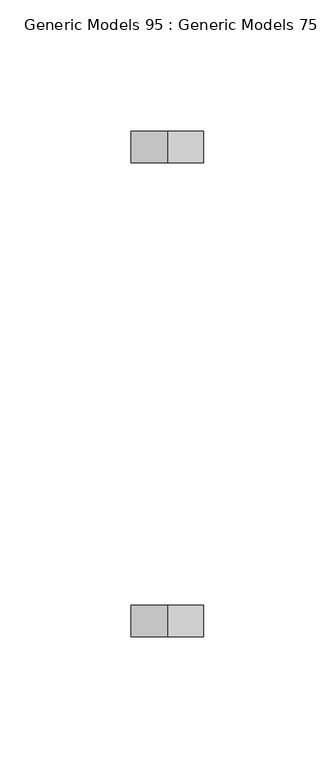
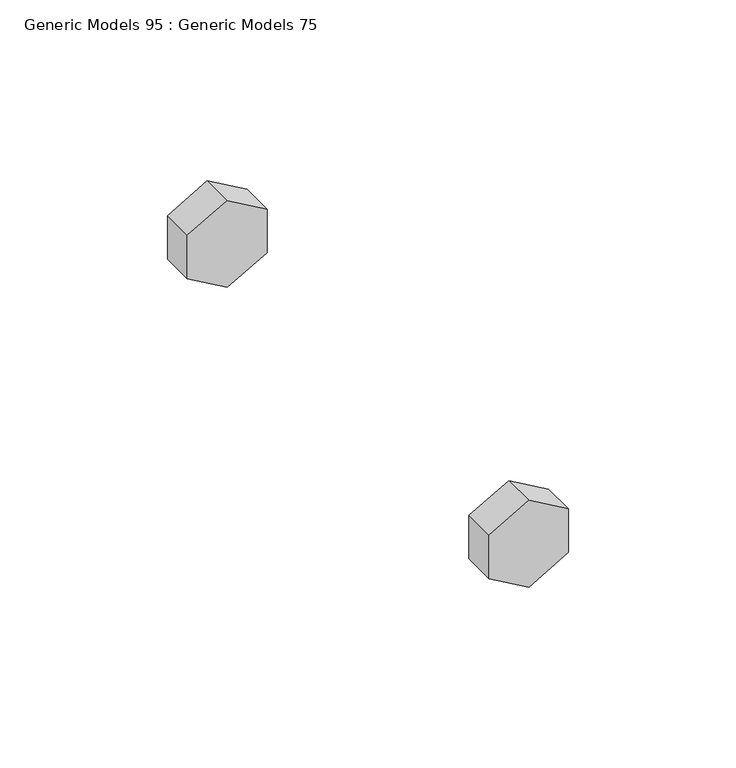
"""IFC4 building model written with IfcOpenShell, lengths in millimetres: proxy geometry, Generic Models 95 : Generic Models 75."""

from ifc_helpers import new_model, si_unit, frame, origin, place, context, project, spatial, polyline, outline, extrude, source, transform, mapped, element, save


def generic_models_95_generic_models_75_713a9572(model_context):
    return source(origin(), model_context, "Body", "SweptSolid", [
        extrude(outline(polyline([(268613.0902933, 31974.4067029), (268597.2537198, 31974.4067029), (268589.335433, 31988.1215778), (268597.2537198, 32001.8364528), (268613.0902933, 32001.8364528), (268621.00858, 31988.1215778), (268613.0902933, 31974.4067029)])), frame((0.0, 36491.5582942, 0.0), z_axis=(0.0, 1.0, 0.0), x_axis=(0.0, 0.0, 1.0)), (0.0, 0.0, 1.0), 11.90625),
        extrude(outline(polyline([(268613.0902933, 31974.4067029), (268597.2537198, 31974.4067029), (268589.335433, 31988.1215778), (268597.2537198, 32001.8364528), (268613.0902933, 32001.8364528), (268621.00858, 31988.1215778), (268613.0902933, 31974.4067029)])), frame((0.0, 36311.3770442, 0.0), z_axis=(0.0, 1.0, 0.0), x_axis=(0.0, 0.0, 1.0)), (0.0, 0.0, 1.0), 11.90625),
    ])


if __name__ == "__main__":
    model = new_model("IFC4")
    model_context = context("Model", 3, world=origin())
    ifc_project = project(units=[si_unit("LENGTHUNIT", "METRE", prefix="MILLI")], contexts=[model_context])
    site = spatial("IfcSite", under=ifc_project)
    building = spatial("IfcBuilding", under=site)
    placement = place(None, origin())
    generic_models_95_generic_models_75_shape = generic_models_95_generic_models_75_713a9572(model_context)
    element("IfcBuildingElementProxy", 1, Name="Generic Models 95 : Generic Models 75", ObjectType="Generic Models 95 : Generic Models 75", at=placement, inside=building, context=model_context, shape_type="MappedRepresentation", body=[
        mapped(generic_models_95_generic_models_75_shape, transform((0.0, 0.0, 0.0), x_axis=(1.0, 0.0, 0.0), y_axis=(0.0, 1.0, 0.0), z_axis=(0.0, 0.0, 1.0))),
    ])
    save(model, "model.ifc")

# Revit data of these elements
# Element 1 (IfcBuildingElementProxy, "Generic Models 95 : Generic Models 75")
#   Materials on its faces: "3/4\" GALV. THRU BOLTS"
# Materials
#   "3/4\" GALV. THRU BOLTS": class "Generic", colour RGB 105 69 171, transparency 0, Cost = 0
